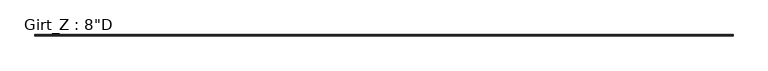
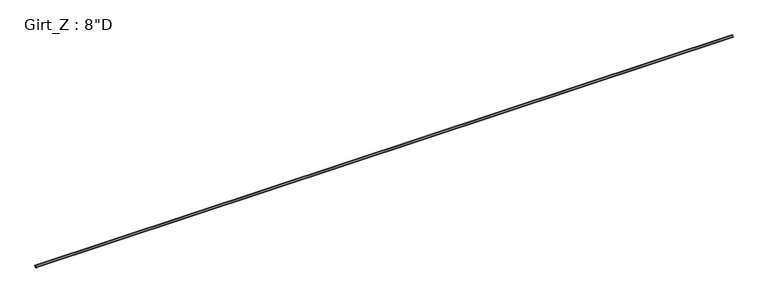
"""IFC4 building model written with IfcOpenShell, lengths in millimetres: beam geometry."""

from ifc_helpers import new_model, si_unit, point, frame, frame_2d, origin, place, context, project, spatial, polyline, circle_curve, trimmed, segment, composite_curve, outline, extrude, source, transform, mapped, element, save


def beam_e7deaa14(model_context):
    return source(origin(), model_context, "Body", "SweptSolid", [
        extrude(outline(composite_curve([segment(polyline([(63.5, 101.6), (75.745104, 87.0068534), (73.6169367, 85.221109), (62.204539, 98.821875), (3.3005807, 98.821875)]), True, "CONTINUOUS"), segment(trimmed(circle_curve(frame_2d((3.3741066, 96.8381931)), 1.9850441), [point((3.3005807, 98.821875))], [point((1.3890625, 96.8381931))], True, "CARTESIAN"), True, "CONTINUOUS"), segment(polyline([(1.3890625, 96.8381931), (1.3890625, -96.8375)]), True, "CONTINUOUS"), segment(trimmed(circle_curve(frame_2d((-3.3734375, -96.8375)), 4.7625), [point((1.3890625, -96.8375))], [point((-3.3734375, -101.6))], False, "CARTESIAN"), True, "CONTINUOUS"), segment(polyline([(-3.3734375, -101.6), (-63.5, -101.6), (-75.745104, -87.0068534), (-73.6169367, -85.221109), (-62.204539, -98.821875), (-3.2694106, -98.821875)]), True, "CONTINUOUS"), segment(trimmed(circle_curve(frame_2d((-3.3748024, -96.8389339)), 1.9857399), [point((-3.2694106, -98.821875))], [point((-1.3890625, -96.8389339))], True, "CARTESIAN"), True, "CONTINUOUS"), segment(polyline([(-1.3890625, -96.8389339), (-1.3890625, 96.8375)]), True, "CONTINUOUS"), segment(trimmed(circle_curve(frame_2d((3.3734375, 96.8375)), 4.7625), [point((-1.3890625, 96.8375))], [point((3.3734375, 101.6))], False, "CARTESIAN"), True, "CONTINUOUS"), segment(polyline([(3.3734375, 101.6), (63.5, 101.6)]), True, "CONTINUOUS")], self_intersect=False)), frame((-40669.2447266, 0.0, 0.0), z_axis=(1.0, 0.0, 0.0), x_axis=(0.0, 1.0, 0.0)), (0.0, 0.0, 1.0), 80870.1769531),
    ])


if __name__ == "__main__":
    model = new_model("IFC4")
    model_context = context("Model", 3, world=origin())
    ifc_project = project(units=[si_unit("LENGTHUNIT", "METRE", prefix="MILLI")], contexts=[model_context])
    site = spatial("IfcSite", under=ifc_project)
    building = spatial("IfcBuilding", under=site)
    placement = place(None, origin())
    beam_shape = beam_e7deaa14(model_context)
    element("IfcBeam", 1, ObjectType="Girt_Z : 8\"D", at=placement, inside=building, context=model_context, shape_type="MappedRepresentation", body=[
        mapped(beam_shape, transform((0.0, 0.0, 0.0), x_axis=(1.0, 0.0, 0.0), y_axis=(0.0, 1.0, 0.0), z_axis=(0.0, 0.0, 1.0))),
    ])
    save(model, "model.ifc")

# Revit data of these elements
# Type "Girt_Z : 8\"D"
#   Web_Thickness = 0' - 0 7/64"
#   Length [instance default] = 10' - 0"
#   Leg_1 = 0' - 2 1/2"
#   Height = 0' - 8"
#   Structural Material [instance default] = none
# Element 1 (IfcBeam, "Girt_Z : 8\"D")
#   Structural Material = Steel
#   Materials on its faces: "Steel"
# Materials
#   "Steel": class "Metal", colour RGB 118 118 114, transparency 0, Description = "Steel, mill finish", Cost = 0
